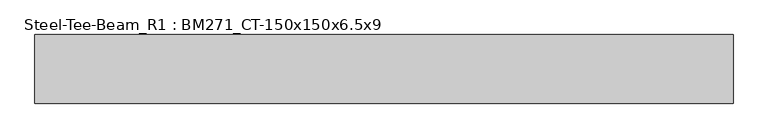
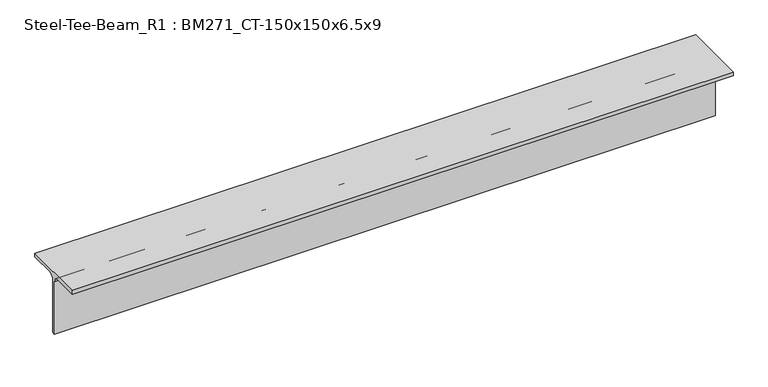
"""IFC4 building model written with IfcOpenShell, lengths in millimetres: member geometry, Steel-Tee-Beam_R1 : BM271_CT-150x150x6.5x9."""

from ifc_helpers import new_model, si_unit, point, frame, frame_2d, origin, place, context, project, spatial, polyline, circle_curve, trimmed, segment, composite_curve, outline, extrude, source, transform, mapped, element, save


def steel_tee_beam_r1_bm271_ct_150x150x6_5x9_ace698d5(model_context):
    return source(origin(), model_context, "Body", "SweptSolid", [
        extrude(outline(composite_curve([segment(polyline([(75.0, 75.0), (75.0, 66.0), (16.25, 66.0)]), True, "CONTINUOUS"), segment(trimmed(circle_curve(frame_2d((16.25, 53.0)), 13.0), [point((16.25, 66.0))], [point((3.25, 53.0))], True, "CARTESIAN"), True, "CONTINUOUS"), segment(polyline([(3.25, 53.0), (3.25, -75.0), (-3.25, -75.0), (-3.25, 53.0)]), True, "CONTINUOUS"), segment(trimmed(circle_curve(frame_2d((-16.25, 53.0)), 13.0), [point((-3.25, 53.0))], [point((-16.25, 66.0))], True, "CARTESIAN"), True, "CONTINUOUS"), segment(polyline([(-16.25, 66.0), (-75.0, 66.0), (-75.0, 75.0), (75.0, 75.0)]), True, "CONTINUOUS")], self_intersect=False)), frame((-719.0402776, 0.0, 0.0), z_axis=(1.0, 0.0, 0.0), x_axis=(0.0, 1.0, 0.0)), (0.0, 0.0, 1.0), 1526.1440409),
    ])


if __name__ == "__main__":
    model = new_model("IFC4")
    model_context = context("Model", 3, world=origin())
    ifc_project = project(units=[si_unit("LENGTHUNIT", "METRE", prefix="MILLI")], contexts=[model_context])
    site = spatial("IfcSite", under=ifc_project)
    building = spatial("IfcBuilding", under=site)
    placement = place(None, origin())
    steel_tee_beam_r1_bm271_ct_150x150x6_5x9_shape = steel_tee_beam_r1_bm271_ct_150x150x6_5x9_ace698d5(model_context)
    element("IfcMember", 1, ObjectType="Steel-Tee-Beam_R1 : BM271_CT-150x150x6.5x9", at=placement, inside=building, context=model_context, shape_type="MappedRepresentation", body=[
        mapped(steel_tee_beam_r1_bm271_ct_150x150x6_5x9_shape, transform((0.0, 0.0, 0.0), x_axis=(1.0, 0.0, 0.0), y_axis=(0.0, 1.0, 0.0), z_axis=(0.0, 0.0, 1.0))),
    ])
    save(model, "model.ifc")

# Revit data of these elements
# Type "Steel-Tee-Beam_R1 : BM271_CT-150x150x6.5x9"
#   Keynote = "CT-150x150x6.5x9"
#   Surface Area = 0.588841 m²/m
#   Section Area = 23.3904 cm²
#   Mass per Unit Length = 18.3614 kg/m
#   Length [instance default] = 1.5240 m
#   bf = 0.1500 m
#   d = 0.1500 m
#   k = 0.0220 m
#   r = 0.0130 m
#   tf = 0.0090 m
#   tw = 0.0065 m
#   hec_material4 [instance default] = none
#   hec_material3 [instance default] = none
#   hec_material2 [instance default] = none
#   hec_material1 [instance default] = none
#   Structural Material [instance default] = Steel, 45-345
#   Assembly Code = ""
# Element 1 (IfcMember, "Steel-Tee-Beam_R1 : BM271_CT-150x150x6.5x9")
#   Structural Material = none
# Materials
#   "Steel, 45-345": class "Metal", colour RGB 189 187 185, transparency 0, Description = "Steel 345 MPa", Cost = 0
